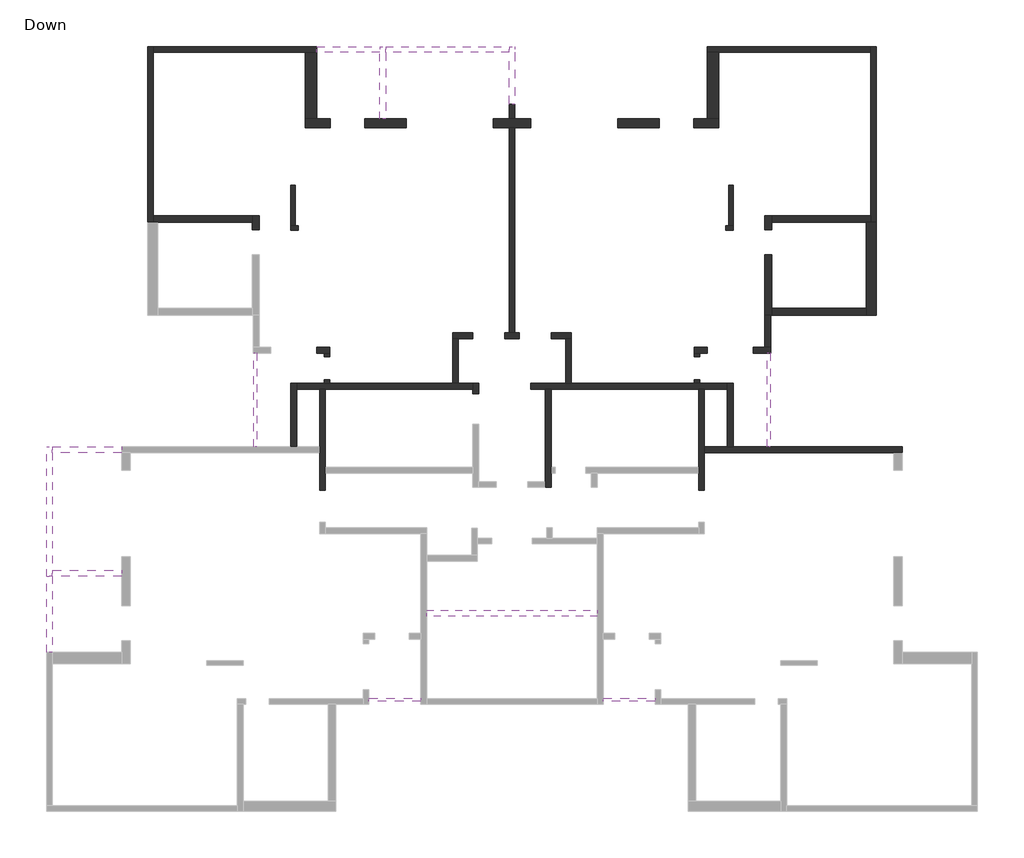
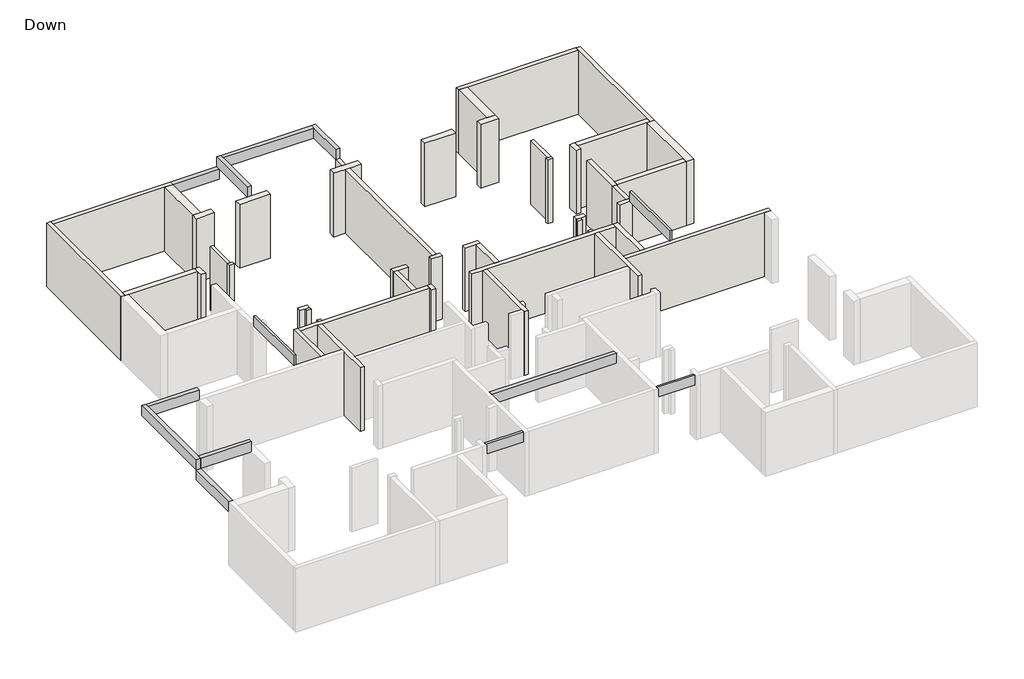
# One storey, part 2 of 2: 46 walls, 13 beams.
"""IFC4 building model written with IfcOpenShell, lengths in millimetres."""

from ifc_helpers import new_model, si_unit, frame, origin, place, context, project, spatial, polyline, outline, extrude, faceted_brep, element, save

model = new_model("IFC4")

# Units and contexts
model_context = context("Model", 3, world=origin())
ifc_project = project(units=[si_unit("LENGTHUNIT", "METRE", prefix="MILLI")], contexts=[model_context])

# Site, building, storey
site = spatial("IfcSite", under=ifc_project)
building = spatial("IfcBuilding", under=site)
storey = spatial("IfcBuildingStorey", under=building, Name="Down", Elevation=0.0)

# Beams
placement = place(None, origin())
element("IfcBeam", 1, ObjectType="Concrete Rectengular Beam : 10/50", at=placement, inside=storey, context=model_context, shape_type="Brep", body=[
    faceted_brep([(-4793.2776511, -8420.9452063, 3180.0), (-4793.2776511, -8520.9452063, 3180.0), (-2993.9832015, -8520.9452063, 3180.0), (-2993.9832015, -8420.9452063, 3180.0), (-4793.2776511, -8520.9452063, 2680.0), (-2993.9832015, -8520.9452063, 2680.0), (-4793.2776511, -8420.9452063, 2680.0), (-2993.9832015, -8420.9452063, 2680.0), (-4793.2776511, -8420.9452063, 2980.0), (-2993.9832015, -8420.9452063, 2980.0)], [[[0, 1, 2, 3]], [[1, 4, 5, 2]], [[4, 6, 7, 5]], [[6, 8, 0, 3, 9, 7]], [[1, 0, 8, 6, 4]], [[3, 2, 5, 7, 9]]]),
])
element("IfcBeam", 2, ObjectType="Concrete Rectengular Beam : 10/50", at=placement, inside=storey, context=model_context, shape_type="Brep", body=[
    faceted_brep([(3308.0864128, -8420.9495778, 3180.0), (3308.0864128, -8520.9495778, 3180.0), (5107.3808625, -8520.9495778, 3180.0), (5107.3808625, -8420.9495778, 3180.0), (3308.0864128, -8520.9495778, 2680.0), (5107.3808625, -8520.9495778, 2680.0), (3308.0864128, -8420.9495778, 2680.0), (5107.3808625, -8420.9495778, 2680.0), (3308.0864128, -8420.9495778, 2980.0), (5107.3808625, -8420.9495778, 2980.0)], [[[0, 1, 2, 3]], [[1, 4, 5, 2]], [[4, 6, 7, 5]], [[6, 8, 0, 3, 9, 7]], [[1, 0, 8, 6, 4]], [[3, 2, 5, 7, 9]]]),
])
element("IfcBeam", 3, ObjectType="Concrete Rectengular Beam : 10/50", at=placement, inside=storey, context=model_context, shape_type="SweptSolid", body=[
    extrude(outline(polyline([(-8674.1337189, 279.007757), (-8774.1337189, 279.007757), (-8774.1337189, 3529.1488671), (-8674.1337189, 3529.1488671), (-8674.1337189, 279.007757)])), frame((0.0, 0.0, 3180.0), z_axis=(0.0, 0.0, 1.0), x_axis=(1.0, 0.0, 0.0)), (0.0, 0.0, 1.0), 500.0),
])
element("IfcBeam", 4, ObjectType="Concrete Rectengular Beam : 10/50", at=placement, inside=storey, context=model_context, shape_type="SweptSolid", body=[
    extrude(outline(polyline([(9086.6847195, 279.007757), (8986.6847195, 279.007757), (8986.6847195, 3529.1488671), (9086.6847195, 3529.1488671), (9086.6847195, 279.007757)])), frame((0.0, 0.0, 3180.0), z_axis=(0.0, 0.0, 1.0), x_axis=(1.0, 0.0, 0.0)), (0.0, 0.0, 1.0), 500.0),
])
element("IfcBeam", 5, ObjectType="Concrete Rectengular Beam : 20/50", at=placement, inside=storey, context=model_context, shape_type="Brep", body=[
    faceted_brep([(57.0516057, 12129.1018304, 3680.0), (57.0516057, 12129.1018304, 3180.0), (257.0516057, 12129.1018304, 3180.0), (257.0516057, 12129.1018304, 3680.0), (257.0516057, 13929.1018304, 3680.0), (257.0516057, 14129.1018304, 3680.0), (57.0516057, 14129.1018304, 3680.0), (57.0516057, 13929.1018304, 3680.0), (257.0516057, 13929.1018304, 3180.0), (257.0516057, 14129.1018304, 3180.0), (57.0516057, 13929.1018304, 3180.0), (57.0516057, 14129.1018304, 3180.0)], [[[0, 1, 2, 3]], [[0, 3, 4, 5, 6, 7]], [[3, 2, 8, 9, 5, 4]], [[2, 1, 10, 11, 9, 8]], [[1, 0, 7, 6, 11, 10]], [[6, 5, 9, 11]]]),
])
element("IfcBeam", 6, ObjectType="Concrete Rectengular Beam : 20/50", at=placement, inside=storey, context=model_context, shape_type="SweptSolid", body=[
    extrude(outline(polyline([(-4213.3152805, 13929.1018304), (-4213.3152805, 14129.1018304), (57.0516057, 14129.1018304), (57.0516057, 13929.1018304), (-4213.3152805, 13929.1018304)])), frame((0.0, 0.0, 3180.0), z_axis=(0.0, 0.0, 1.0), x_axis=(1.0, 0.0, 0.0)), (0.0, 0.0, 1.0), 500.0),
])
element("IfcBeam", 7, ObjectType="Concrete Rectengular Beam : 20/50", at=placement, inside=storey, context=model_context, shape_type="Brep", body=[
    faceted_brep([(-4213.3152805, 11629.007757, 3680.0), (-4413.3152805, 11629.007757, 3680.0), (-4413.3152805, 11629.007757, 3180.0), (-4213.3152805, 11629.007757, 3180.0), (-4213.3152805, 14129.1018304, 3680.0), (-4213.3152805, 14129.1018304, 3180.0), (-4413.3152805, 14129.1018304, 3180.0), (-4413.3152805, 14129.1018304, 3680.0), (-4213.3152805, 13929.1018304, 3680.0), (-4213.3152805, 13929.1018304, 3180.0)], [[[0, 1, 2, 3]], [[4, 5, 6, 7]], [[1, 0, 8, 4, 7]], [[2, 1, 7, 6]], [[3, 2, 6, 5, 9]], [[0, 3, 9, 5, 4, 8]]]),
])
element("IfcBeam", 8, ObjectType="Concrete Rectengular Beam : 20/50", at=placement, inside=storey, context=model_context, shape_type="Brep", body=[
    faceted_brep([(-15942.7132109, -4192.3939363, 3180.0), (-15742.7132109, -4192.3939363, 3180.0), (-15742.7132109, -4192.3939363, 2680.0), (-15942.7132109, -4192.3939363, 2680.0), (-15942.7132109, -4192.3939363, 2980.0), (-15942.7132109, -6821.2744631, 3180.0), (-15742.7132109, -6821.2744631, 3180.0), (-15742.7132109, -6821.2744631, 2680.0), (-15942.7132109, -6821.2744631, 2680.0)], [[[0, 1, 2, 3, 4]], [[1, 0, 5, 6]], [[2, 1, 6, 7]], [[3, 2, 7, 8]], [[0, 4, 3, 8, 5]], [[6, 5, 8, 7]]]),
])
element("IfcBeam", 9, ObjectType="Concrete Rectengular Beam : 20/50", at=placement, inside=storey, context=model_context, shape_type="SweptSolid", body=[
    extrude(outline(polyline([(-13342.9013576, -3992.3939363), (-13342.9013576, -4192.3939363), (-15742.7132109, -4192.3939363), (-15742.7132109, -3992.3939363), (-13342.9013576, -3992.3939363)])), frame((0.0, 0.0, 3180.0), z_axis=(0.0, 0.0, 1.0), x_axis=(1.0, 0.0, 0.0)), (0.0, 0.0, 1.0), 500.0),
])
element("IfcBeam", 10, ObjectType="Concrete Rectengular Beam : 20/50", at=placement, inside=storey, context=model_context, shape_type="Brep", body=[
    faceted_brep([(-15942.7132109, -4192.3939363, 3680.0), (-15942.7132109, -4192.3939363, 3180.0), (-15742.7132109, -4192.3939363, 3180.0), (-15742.7132109, -4192.3939363, 3680.0), (-15742.7132109, -3992.3939363, 3680.0), (-15742.7132109, 79.007757, 3680.0), (-15742.7132109, 279.007757, 3680.0), (-15942.7132109, 279.007757, 3680.0), (-15742.7132109, -3992.3939363, 3180.0), (-15742.7132109, 79.007757, 3180.0), (-15742.7132109, 279.007757, 3180.0), (-15942.7132109, 279.007757, 3180.0)], [[[0, 1, 2, 3]], [[0, 3, 4, 5, 6, 7]], [[3, 2, 8, 9, 10, 6, 5, 4]], [[2, 1, 11, 10, 9, 8]], [[1, 0, 7, 11]], [[7, 6, 10, 11]]]),
])
element("IfcBeam", 11, ObjectType="Concrete Rectengular Beam : 20/50", at=placement, inside=storey, context=model_context, shape_type="SweptSolid", body=[
    extrude(outline(polyline([(-13343.4657979, 279.007757), (-13343.4657979, 79.007757), (-15742.7132109, 79.007757), (-15742.7132109, 279.007757), (-13343.4657979, 279.007757)])), frame((0.0, 0.0, 3180.0), z_axis=(0.0, 0.0, 1.0), x_axis=(1.0, 0.0, 0.0)), (0.0, 0.0, 1.0), 500.0),
])
element("IfcBeam", 12, ObjectType="Concrete Rectengular Beam : 20/50", at=placement, inside=storey, context=model_context, shape_type="Brep", body=[
    faceted_brep([(-4413.3152805, 13929.1018304, 3180.0), (-4413.3152805, 13929.1018304, 2680.0), (-4413.3152805, 14129.1018304, 2680.0), (-4413.3152805, 14129.1018304, 2980.0), (-4413.3152805, 14129.1018304, 3180.0), (-6593.4657979, 14129.1018304, 3180.0), (-6593.4657979, 13929.3370139, 3180.0), (-6593.4657979, 13929.1018304, 3180.0), (-6593.4657979, 14129.1018304, 2680.0), (-6593.4657979, 13929.1018304, 2680.0)], [[[0, 1, 2, 3, 4]], [[0, 4, 5, 6, 7]], [[4, 3, 2, 8, 5]], [[2, 1, 9, 8]], [[1, 0, 7, 9]], [[5, 8, 9, 7, 6]]]),
])
element("IfcBeam", 13, ObjectType="Concrete Rectengular Beam : 20/50", at=placement, inside=storey, context=model_context, shape_type="Brep", body=[
    faceted_brep([(-2793.9832015, -5372.4503803, 3180.0), (-2793.9832015, -5572.4503803, 3180.0), (3108.0864128, -5572.4503803, 3180.0), (3108.0864128, -5372.4503803, 3180.0), (-2793.9832015, -5572.4503803, 2680.0), (3108.0864128, -5572.4503803, 2680.0), (-2793.9832015, -5372.4503803, 2680.0), (3108.0864128, -5372.4503803, 2680.0), (-2793.9832015, -5372.4503803, 2980.0), (3108.0864128, -5372.4503803, 2980.0)], [[[0, 1, 2, 3]], [[1, 4, 5, 2]], [[4, 6, 7, 5]], [[6, 8, 0, 3, 9, 7]], [[1, 0, 8, 6, 4]], [[3, 2, 5, 7, 9]]]),
])

# Walls
element("IfcWall", 14, ObjectType="15", at=placement, inside=storey, context=model_context, shape_type="Brep", body=[
    faceted_brep([(-7241.1610001, 7927.5496197, 0.0), (-7340.9258167, 7927.5496197, 0.0), (-7490.9258167, 7927.5496197, 0.0), (-7490.9258167, 7927.5496197, 3180.0), (-7340.9258167, 7927.5496197, 3180.0), (-7241.1610001, 7927.5496197, 3180.0), (-7241.1610001, 7927.5496197, 2980.0), (-7241.1610001, 7777.5496197, 0.0), (-7241.1610001, 7777.5496197, 2980.0), (-7241.1610001, 7777.5496197, 3180.0), (-7490.9258167, 7777.5496197, 3180.0), (-7490.9258167, 7777.5496197, 2980.0), (-7490.9258167, 7777.5496197, 0.0)], [[[0, 1, 2, 3, 4, 5, 6]], [[7, 8, 9, 10, 11, 12]], [[2, 1, 0, 7, 12]], [[5, 4, 3, 10, 9]], [[0, 6, 5, 9, 8, 7]], [[3, 2, 12, 11, 10]]]),
])
element("IfcWall", 15, ObjectType="15", at=placement, inside=storey, context=model_context, shape_type="Brep", body=[
    faceted_brep([(-7340.9258167, 7927.5496197, 0.0), (-7340.9258167, 9328.7725736, 0.0), (-7340.9258167, 9328.7725736, 2980.0), (-7340.9258167, 9328.7725736, 3180.0), (-7340.9258167, 7927.5496197, 3180.0), (-7340.9258167, 7927.5496197, 2980.0), (-7490.9258167, 7927.5496197, 0.0), (-7490.9258167, 7927.5496197, 3180.0), (-7490.9258167, 9328.7725736, 3180.0), (-7490.9258167, 9328.7725736, 2980.0), (-7490.9258167, 9328.7725736, 0.0)], [[[0, 1, 2, 3, 4, 5]], [[6, 7, 8, 9, 10]], [[1, 0, 6, 10]], [[3, 2, 1, 10, 9, 8]], [[4, 3, 8, 7]], [[0, 5, 4, 7, 6]]]),
])
element("IfcWall", 16, ObjectType="15", at=placement, inside=storey, context=model_context, shape_type="Brep", body=[
    faceted_brep([(7555.2642115, 7777.5496197, 0.0), (7805.0290281, 7777.5496197, 0.0), (7805.0290281, 7777.5496197, 2980.0), (7805.0290281, 7777.5496197, 3180.0), (7555.2642115, 7777.5496197, 3180.0), (7555.2642115, 7777.5496197, 2980.0), (7555.2642115, 7927.5496197, 0.0), (7555.2642115, 7927.5496197, 2980.0), (7555.2642115, 7927.5496197, 3180.0), (7655.0290281, 7927.5496197, 3180.0), (7805.0290281, 7927.5496197, 3180.0), (7805.0290281, 7927.5496197, 0.0), (7655.0290281, 7927.5496197, 0.0)], [[[0, 1, 2, 3, 4, 5]], [[6, 7, 8, 9, 10, 11, 12]], [[1, 0, 6, 12, 11]], [[4, 3, 10, 9, 8]], [[0, 5, 4, 8, 7, 6]], [[3, 2, 1, 11, 10]]]),
])
element("IfcWall", 17, ObjectType="15", at=placement, inside=storey, context=model_context, shape_type="Brep", body=[
    faceted_brep([(7805.0290281, 7927.5496197, 0.0), (7805.0290281, 9328.7725736, 0.0), (7805.0290281, 9328.7725736, 2980.0), (7805.0290281, 9328.7725736, 3180.0), (7805.0290281, 7927.5496197, 3180.0), (7655.0290281, 7927.5496197, 0.0), (7655.0290281, 7927.5496197, 2980.0), (7655.0290281, 7927.5496197, 3180.0), (7655.0290281, 9328.7725736, 3180.0), (7655.0290281, 9328.7725736, 2980.0), (7655.0290281, 9328.7725736, 0.0)], [[[0, 1, 2, 3, 4]], [[5, 6, 7, 8, 9, 10]], [[1, 0, 5, 10]], [[3, 2, 1, 10, 9, 8]], [[4, 3, 8, 7]], [[0, 4, 7, 6, 5]]]),
])
element("IfcWall", 18, ObjectType="20", at=placement, inside=storey, context=model_context, shape_type="Brep", body=[
    faceted_brep([(-12443.8891281, 14129.3370139, 0.0), (-12443.8891281, 8055.2636366, 0.0), (-12443.8891281, 8055.2636366, 3180.0), (-12443.8891281, 14129.3370139, 3180.0), (-12243.8891281, 14129.3370139, 0.0), (-12243.8891281, 14129.3370139, 3180.0), (-12243.8891281, 13929.3370139, 3180.0), (-12243.8891281, 8285.2636366, 3180.0), (-12243.8891281, 8055.2636366, 3180.0), (-12243.8891281, 8055.2636366, 0.0), (-12243.8891281, 8285.2636366, 0.0), (-12243.8891281, 13929.3370139, 0.0)], [[[0, 1, 2, 3]], [[4, 5, 6, 7, 8, 9, 10, 11]], [[1, 0, 4, 11, 10, 9]], [[3, 2, 8, 7, 6, 5]], [[2, 1, 9, 8]], [[0, 3, 5, 4]]]),
])
element("IfcWall", 19, ObjectType="20", at=placement, inside=storey, context=model_context, shape_type="Brep", body=[
    faceted_brep([(-6593.4657979, 3529.1488671, 0.0), (-6344.7357885, 3529.1488671, 0.0), (-6144.7357885, 3529.1488671, 0.0), (-6144.7357885, 3529.1488671, 3180.0), (-6344.7357885, 3529.1488671, 3180.0), (-6593.4657979, 3529.1488671, 3180.0), (-6593.4657979, 3529.1488671, 2980.0), (-6593.4657979, 3729.1488671, 0.0), (-6593.4657979, 3729.1488671, 2980.0), (-6593.4657979, 3729.1488671, 3180.0), (-6144.7357885, 3729.1488671, 3180.0), (-6144.7357885, 3729.1488671, 2980.0), (-6144.7357885, 3729.1488671, 0.0)], [[[0, 1, 2, 3, 4, 5, 6]], [[7, 8, 9, 10, 11, 12]], [[2, 1, 0, 7, 12]], [[5, 4, 3, 10, 9]], [[0, 6, 5, 9, 8, 7]], [[3, 2, 12, 11, 10]]]),
])
element("IfcWall", 20, ObjectType="20", at=placement, inside=storey, context=model_context, shape_type="Brep", body=[
    faceted_brep([(-6344.7357885, 3529.1488671, 0.0), (-6344.7357885, 3397.9165059, 0.0), (-6344.7357885, 3397.9165059, 2980.0), (-6344.7357885, 3397.9165059, 3180.0), (-6344.7357885, 3529.1488671, 3180.0), (-6344.7357885, 3529.1488671, 2980.0), (-6144.7357885, 3529.1488671, 0.0), (-6144.7357885, 3529.1488671, 3180.0), (-6144.7357885, 3397.9165059, 3180.0), (-6144.7357885, 3397.9165059, 2980.0), (-6144.7357885, 3397.9165059, 0.0)], [[[0, 1, 2, 3, 4, 5]], [[6, 7, 8, 9, 10]], [[1, 0, 6, 10]], [[3, 2, 1, 10, 9, 8]], [[4, 3, 8, 7]], [[0, 5, 4, 7, 6]]]),
])
element("IfcWall", 21, ObjectType="20", at=placement, inside=storey, context=model_context, shape_type="Brep", body=[
    faceted_brep([(-6344.7357885, 2597.8224325, 0.0), (-6344.7357885, 2479.2899772, 0.0), (-6344.7357885, 2479.2899772, 2980.0), (-6344.7357885, 2479.2899772, 3180.0), (-6344.7357885, 2597.8224325, 3180.0), (-6344.7357885, 2597.8224325, 2980.0), (-6144.7357885, 2597.8224325, 0.0), (-6144.7357885, 2597.8224325, 2980.0), (-6144.7357885, 2597.8224325, 3180.0), (-6144.7357885, 2479.2899772, 3180.0), (-6144.7357885, 2479.2899772, 2980.0), (-6144.7357885, 2479.2899772, 0.0)], [[[0, 1, 2, 3, 4, 5]], [[6, 7, 8, 9, 10, 11]], [[1, 0, 6, 11]], [[4, 3, 9, 8]], [[0, 5, 4, 8, 7, 6]], [[3, 2, 1, 11, 10, 9]]]),
])
element("IfcWall", 22, ObjectType="20", at=placement, inside=storey, context=model_context, shape_type="Brep", body=[
    faceted_brep([(-7293.0424677, 2279.2899772, 0.0), (-6495.0180086, 2279.2899772, 0.0), (-6295.0180086, 2279.2899772, 0.0), (-1194.9239352, 2279.2899772, 0.0), (-1194.9239352, 2279.2899772, 3180.0), (-6295.0180086, 2279.2899772, 3180.0), (-6495.0180086, 2279.2899772, 3180.0), (-7293.0424677, 2279.2899772, 3180.0), (-7293.0424677, 2479.2899772, 0.0), (-7293.0424677, 2479.2899772, 3180.0), (-6344.7357885, 2479.2899772, 3180.0), (-6144.7357885, 2479.2899772, 3180.0), (-1894.500605, 2479.2899772, 3180.0), (-1694.500605, 2479.2899772, 3180.0), (-1194.9239352, 2479.2899772, 3180.0), (-1194.9239352, 2479.2899772, 0.0), (-1694.500605, 2479.2899772, 0.0), (-1894.500605, 2479.2899772, 0.0), (-6144.7357885, 2479.2899772, 0.0), (-6344.7357885, 2479.2899772, 0.0)], [[[0, 1, 2, 3, 4, 5, 6, 7]], [[8, 9, 10, 11, 12, 13, 14, 15, 16, 17, 18, 19]], [[3, 2, 1, 0, 8, 19, 18, 17, 16, 15]], [[7, 6, 5, 4, 14, 13, 12, 11, 10, 9]], [[4, 3, 15, 14]], [[0, 7, 9, 8]]]),
])
element("IfcWall", 23, ObjectType="20", at=placement, inside=storey, context=model_context, shape_type="Brep", body=[
    faceted_brep([(-1194.9239352, 2479.2899772, 0.0), (-1194.9239352, 2279.2899772, 0.0), (-1194.9239352, 2127.9259132, 0.0), (-1194.9239352, 2127.9259132, 2980.0), (-1194.9239352, 2127.9259132, 3180.0), (-1194.9239352, 2279.2899772, 3180.0), (-1194.9239352, 2479.2899772, 3180.0), (-994.9239352, 2479.2899772, 0.0), (-994.9239352, 2479.2899772, 2980.0), (-994.9239352, 2479.2899772, 3180.0), (-994.9239352, 2127.9259132, 3180.0), (-994.9239352, 2127.9259132, 2980.0), (-994.9239352, 2127.9259132, 0.0), (-1133.7398977, 2479.2899772, 3180.0)], [[[0, 1, 2, 3, 4, 5, 6]], [[7, 8, 9, 10, 11, 12]], [[2, 1, 0, 7, 12]], [[4, 3, 2, 12, 11, 10]], [[6, 5, 4, 10, 9, 13]], [[0, 6, 13, 9, 8, 7]]]),
])
element("IfcWall", 24, ObjectType="20", at=placement, inside=storey, context=model_context, shape_type="Brep", body=[
    faceted_brep([(-6295.0180086, -1222.7326004, 0.0), (-6295.0180086, -621.6037199, 0.0), (-6295.0180086, -421.6037199, 0.0), (-6295.0180086, 2279.2899772, 0.0), (-6295.0180086, 2279.2899772, 3180.0), (-6295.0180086, -421.6037199, 3180.0), (-6295.0180086, -621.6037199, 3180.0), (-6295.0180086, -1222.7326004, 3180.0), (-6295.0180086, -1222.7326004, 2980.0), (-6495.0180086, -1222.7326004, 0.0), (-6495.0180086, -1222.7326004, 2980.0), (-6495.0180086, -1222.7326004, 3180.0), (-6495.0180086, 79.007757, 3180.0), (-6495.0180086, 279.007757, 3180.0), (-6495.0180086, 2279.2899772, 3180.0), (-6495.0180086, 2279.2899772, 0.0), (-6495.0180086, 279.007757, 0.0), (-6495.0180086, 79.007757, 0.0)], [[[0, 1, 2, 3, 4, 5, 6, 7, 8]], [[9, 10, 11, 12, 13, 14, 15, 16, 17]], [[3, 2, 1, 0, 9, 17, 16, 15]], [[7, 6, 5, 4, 14, 13, 12, 11]], [[0, 8, 7, 11, 10, 9]], [[4, 3, 15, 14]]]),
])
element("IfcWall", 25, ObjectType="20", at=placement, inside=storey, context=model_context, shape_type="Brep", body=[
    faceted_brep([(-7493.0424677, 2479.2899772, 0.0), (-7493.0424677, 279.007757, 0.0), (-7493.0424677, 279.007757, 2980.0), (-7493.0424677, 279.007757, 3180.0), (-7493.0424677, 2479.2899772, 3180.0), (-7493.0424677, 2479.2899772, 2980.0), (-7293.0424677, 2479.2899772, 0.0), (-7293.0424677, 2479.2899772, 3180.0), (-7293.0424677, 2279.2899772, 3180.0), (-7293.0424677, 279.007757, 3180.0), (-7293.0424677, 279.007757, 0.0), (-7293.0424677, 2279.2899772, 0.0)], [[[0, 1, 2, 3, 4, 5]], [[6, 7, 8, 9, 10, 11]], [[1, 0, 6, 11, 10]], [[4, 3, 9, 8, 7]], [[3, 2, 1, 10, 9]], [[0, 5, 4, 7, 6]]]),
])
element("IfcWall", 26, ObjectType="20", at=placement, inside=storey, context=model_context, shape_type="Brep", body=[
    faceted_brep([(-12243.8891281, 13929.3370139, 0.0), (-6993.4657979, 13929.3370139, 0.0), (-6593.4657979, 13929.3370139, 0.0), (-6593.4657979, 13929.3370139, 3180.0), (-6993.4657979, 13929.3370139, 3180.0), (-12243.8891281, 13929.3370139, 3180.0), (-12243.8891281, 13929.3370139, 2980.0), (-12243.8891281, 14129.3370139, 0.0), (-12243.8891281, 14129.3370139, 3180.0), (-6593.4657979, 14129.3370139, 3180.0), (-6593.4657979, 14129.3370139, 0.0), (-6593.4657979, 14129.1018304, 3180.0)], [[[0, 1, 2, 3, 4, 5, 6]], [[7, 8, 9, 10]], [[2, 1, 0, 7, 10]], [[5, 4, 3, 11, 9, 8]], [[0, 6, 5, 8, 7]], [[3, 2, 10, 9, 11]]]),
])
element("IfcWall", 27, ObjectType="20", at=placement, inside=storey, context=model_context, shape_type="Brep", body=[
    faceted_brep([(57.0516057, 12129.1018304, 0.0), (57.0516057, 11629.007757, 0.0), (57.0516057, 11629.007757, 2980.0), (57.0516057, 11629.007757, 3180.0), (57.0516057, 12129.1018304, 3180.0), (57.0516057, 12129.1018304, 2980.0), (257.0516057, 12129.1018304, 0.0), (257.0516057, 12129.1018304, 2980.0), (257.0516057, 12129.1018304, 3180.0), (257.0516057, 11629.007757, 3180.0), (257.0516057, 11629.007757, 2980.0), (257.0516057, 11629.007757, 0.0)], [[[0, 1, 2, 3, 4, 5]], [[6, 7, 8, 9, 10, 11]], [[1, 0, 6, 11]], [[4, 3, 9, 8]], [[0, 5, 4, 8, 7, 6]], [[3, 2, 1, 11, 10, 9]]]),
])
element("IfcWall", 28, ObjectType="20", at=placement, inside=storey, context=model_context, shape_type="Brep", body=[
    faceted_brep([(57.0516057, 11329.007757, 0.0), (57.0516057, 4229.007757, 0.0), (57.0516057, 4229.007757, 2980.0), (57.0516057, 4229.007757, 3180.0), (57.0516057, 11329.007757, 3180.0), (57.0516057, 11329.007757, 2980.0), (257.0516057, 11329.007757, 0.0), (257.0516057, 11329.007757, 2980.0), (257.0516057, 11329.007757, 3180.0), (257.0516057, 4229.007757, 3180.0), (257.0516057, 4229.007757, 2980.0), (257.0516057, 4229.007757, 0.0)], [[[0, 1, 2, 3, 4, 5]], [[6, 7, 8, 9, 10, 11]], [[1, 0, 6, 11]], [[4, 3, 9, 8]], [[0, 5, 4, 8, 7, 6]], [[3, 2, 1, 11, 10, 9]]]),
])
element("IfcWall", 29, ObjectType="20", at=placement, inside=storey, context=model_context, shape_type="Brep", body=[
    faceted_brep([(407.3338258, 4229.007757, 0.0), (257.0516057, 4229.007757, 0.0), (57.0516057, 4229.007757, 0.0), (-93.2306144, 4229.007757, 0.0), (-93.2306144, 4229.007757, 2980.0), (-93.2306144, 4229.007757, 3180.0), (57.0516057, 4229.007757, 3180.0), (257.0516057, 4229.007757, 3180.0), (407.3338258, 4229.007757, 3180.0), (407.3338258, 4229.007757, 2980.0), (407.3338258, 4029.007757, 0.0), (407.3338258, 4029.007757, 2980.0), (407.3338258, 4029.007757, 3180.0), (-93.2306144, 4029.007757, 3180.0), (-93.2306144, 4029.007757, 2980.0), (-93.2306144, 4029.007757, 0.0)], [[[0, 1, 2, 3, 4, 5, 6, 7, 8, 9]], [[10, 11, 12, 13, 14, 15]], [[3, 2, 1, 0, 10, 15]], [[5, 4, 3, 15, 14, 13]], [[8, 7, 6, 5, 13, 12]], [[0, 9, 8, 12, 11, 10]]]),
])
element("IfcWall", 30, ObjectType="20", at=placement, inside=storey, context=model_context, shape_type="Brep", body=[
    faceted_brep([(-1193.8891281, 4228.6785002, 0.0), (-1894.500605, 4228.6785002, 0.0), (-1894.500605, 4228.6785002, 2980.0), (-1894.500605, 4228.6785002, 3180.0), (-1193.8891281, 4228.6785002, 3180.0), (-1193.8891281, 4228.6785002, 2980.0), (-1193.8891281, 4028.6785002, 0.0), (-1193.8891281, 4028.6785002, 3180.0), (-1694.500605, 4028.6785002, 3180.0), (-1894.500605, 4028.6785002, 3180.0), (-1894.500605, 4028.6785002, 0.0), (-1694.500605, 4028.6785002, 0.0), (-1193.8891281, 4029.007757, 3180.0)], [[[0, 1, 2, 3, 4, 5]], [[6, 7, 8, 9, 10, 11]], [[1, 0, 6, 11, 10]], [[4, 3, 9, 8, 7, 12]], [[0, 5, 4, 12, 7, 6]], [[3, 2, 1, 10, 9]]]),
])
element("IfcWall", 31, ObjectType="20", at=placement, inside=storey, context=model_context, shape_type="Brep", body=[
    faceted_brep([(-1894.500605, 4028.6785002, 0.0), (-1894.500605, 2479.2899772, 0.0), (-1894.500605, 2479.2899772, 2980.0), (-1894.500605, 2479.2899772, 3180.0), (-1894.500605, 4028.6785002, 3180.0), (-1694.500605, 4028.6785002, 0.0), (-1694.500605, 4028.6785002, 3180.0), (-1694.500605, 2479.2899772, 3180.0), (-1694.500605, 2479.2899772, 0.0)], [[[0, 1, 2, 3, 4]], [[5, 6, 7, 8]], [[1, 0, 5, 8]], [[4, 3, 7, 6]], [[0, 4, 6, 5]], [[3, 2, 1, 8, 7]]]),
])
element("IfcWall", 32, ObjectType="20", at=placement, inside=storey, context=model_context, shape_type="Brep", body=[
    faceted_brep([(12557.9923395, 14129.3370139, 0.0), (12557.9923395, 13929.3370139, 0.0), (12557.9923395, 8285.2636366, 0.0), (12557.9923395, 8055.2636366, 0.0), (12557.9923395, 8055.2636366, 3180.0), (12557.9923395, 8285.2636366, 3180.0), (12557.9923395, 13929.3370139, 3180.0), (12557.9923395, 14129.3370139, 3180.0), (12757.9923395, 14129.3370139, 0.0), (12757.9923395, 14129.3370139, 3180.0), (12757.9923395, 8055.2636366, 3180.0), (12757.9923395, 8055.2636366, 0.0)], [[[0, 1, 2, 3, 4, 5, 6, 7]], [[8, 9, 10, 11]], [[3, 2, 1, 0, 8, 11]], [[7, 6, 5, 4, 10, 9]], [[4, 3, 11, 10]], [[0, 7, 9, 8]]]),
])
element("IfcWall", 33, ObjectType="20", at=placement, inside=storey, context=model_context, shape_type="Brep", body=[
    faceted_brep([(8907.8041927, 4828.7725736, 0.0), (8907.8041927, 3729.1488671, 0.0), (8907.8041927, 3729.1488671, 2980.0), (8907.8041927, 3729.1488671, 3180.0), (8907.8041927, 4828.7725736, 3180.0), (9107.8041927, 4828.7725736, 0.0), (9107.8041927, 4828.7725736, 3180.0), (9107.8041927, 3729.1488671, 3180.0), (9107.8041927, 3729.1488671, 0.0)], [[[0, 1, 2, 3, 4]], [[5, 6, 7, 8]], [[1, 0, 5, 8]], [[4, 3, 7, 6]], [[0, 4, 6, 5]], [[3, 2, 1, 8, 7]]]),
])
element("IfcWall", 34, ObjectType="20", at=placement, inside=storey, context=model_context, shape_type="Brep", body=[
    faceted_brep([(9107.8041927, 3729.1488671, 0.0), (8907.8041927, 3729.1488671, 0.0), (8507.757156, 3729.1488671, 0.0), (8507.757156, 3729.1488671, 2980.0), (8507.757156, 3729.1488671, 3180.0), (8907.8041927, 3729.1488671, 3180.0), (9107.8041927, 3729.1488671, 3180.0), (9107.8041927, 3529.1488671, 0.0), (9107.8041927, 3529.1488671, 3180.0), (9086.6847195, 3529.1488671, 3180.0), (8507.757156, 3529.1488671, 3180.0), (8507.757156, 3529.1488671, 2980.0), (8507.757156, 3529.1488671, 0.0)], [[[0, 1, 2, 3, 4, 5, 6]], [[7, 8, 9, 10, 11, 12]], [[2, 1, 0, 7, 12]], [[4, 3, 2, 12, 11, 10]], [[6, 5, 4, 10, 9, 8]], [[0, 6, 8, 7]]]),
])
element("IfcWall", 35, ObjectType="20", at=placement, inside=storey, context=model_context, shape_type="Brep", body=[
    faceted_brep([(6907.5690093, 3729.1488671, 0.0), (6458.8389999, 3729.1488671, 0.0), (6458.8389999, 3729.1488671, 2980.0), (6458.8389999, 3729.1488671, 3180.0), (6907.5690093, 3729.1488671, 3180.0), (6907.5690093, 3729.1488671, 2980.0), (6907.5690093, 3529.1488671, 0.0), (6907.5690093, 3529.1488671, 2980.0), (6907.5690093, 3529.1488671, 3180.0), (6658.8389999, 3529.1488671, 3180.0), (6458.8389999, 3529.1488671, 3180.0), (6458.8389999, 3529.1488671, 0.0), (6658.8389999, 3529.1488671, 0.0)], [[[0, 1, 2, 3, 4, 5]], [[6, 7, 8, 9, 10, 11, 12]], [[1, 0, 6, 12, 11]], [[4, 3, 10, 9, 8]], [[0, 5, 4, 8, 7, 6]], [[3, 2, 1, 11, 10]]]),
])
element("IfcWall", 36, ObjectType="20", at=placement, inside=storey, context=model_context, shape_type="Brep", body=[
    faceted_brep([(6458.8389999, 3529.1488671, 0.0), (6458.8389999, 3397.9165059, 0.0), (6458.8389999, 3397.9165059, 2980.0), (6458.8389999, 3397.9165059, 3180.0), (6458.8389999, 3529.1488671, 3180.0), (6658.8389999, 3529.1488671, 0.0), (6658.8389999, 3529.1488671, 2980.0), (6658.8389999, 3529.1488671, 3180.0), (6658.8389999, 3397.9165059, 3180.0), (6658.8389999, 3397.9165059, 2980.0), (6658.8389999, 3397.9165059, 0.0)], [[[0, 1, 2, 3, 4]], [[5, 6, 7, 8, 9, 10]], [[1, 0, 5, 10]], [[3, 2, 1, 10, 9, 8]], [[4, 3, 8, 7]], [[0, 4, 7, 6, 5]]]),
])
element("IfcWall", 37, ObjectType="20", at=placement, inside=storey, context=model_context, shape_type="Brep", body=[
    faceted_brep([(6458.8389999, 2597.8224325, 0.0), (6458.8389999, 2479.2899772, 0.0), (6458.8389999, 2479.2899772, 2980.0), (6458.8389999, 2479.2899772, 3180.0), (6458.8389999, 2597.8224325, 3180.0), (6458.8389999, 2597.8224325, 2980.0), (6658.8389999, 2597.8224325, 0.0), (6658.8389999, 2597.8224325, 2980.0), (6658.8389999, 2597.8224325, 3180.0), (6658.8389999, 2479.2899772, 3180.0), (6658.8389999, 2479.2899772, 2980.0), (6658.8389999, 2479.2899772, 0.0)], [[[0, 1, 2, 3, 4, 5]], [[6, 7, 8, 9, 10, 11]], [[1, 0, 6, 11]], [[4, 3, 9, 8]], [[0, 5, 4, 8, 7, 6]], [[3, 2, 1, 11, 10, 9]]]),
])
element("IfcWall", 38, ObjectType="20", at=placement, inside=storey, context=model_context, shape_type="Brep", body=[
    faceted_brep([(7607.1456791, 2479.2899772, 0.0), (6658.8389999, 2479.2899772, 0.0), (6458.8389999, 2479.2899772, 0.0), (2208.6038164, 2479.2899772, 0.0), (2008.6038164, 2479.2899772, 0.0), (806.3460554, 2479.2899772, 0.0), (806.3460554, 2479.2899772, 2980.0), (806.3460554, 2479.2899772, 3180.0), (1446.2601023, 2479.2899772, 3180.0), (2008.6038164, 2479.2899772, 3180.0), (2208.6038164, 2479.2899772, 3180.0), (6458.8389999, 2479.2899772, 3180.0), (6658.8389999, 2479.2899772, 3180.0), (7607.1456791, 2479.2899772, 3180.0), (7607.1456791, 2279.2899772, 0.0), (7607.1456791, 2279.2899772, 3180.0), (6809.12122, 2279.2899772, 3180.0), (6609.12122, 2279.2899772, 3180.0), (1509.0271466, 2279.2899772, 3180.0), (1309.0271466, 2279.2899772, 3180.0), (806.3460554, 2279.2899772, 3180.0), (806.3460554, 2279.2899772, 2980.0), (806.3460554, 2279.2899772, 0.0), (1309.0271466, 2279.2899772, 0.0), (1509.0271466, 2279.2899772, 0.0), (6609.12122, 2279.2899772, 0.0), (6809.12122, 2279.2899772, 0.0)], [[[0, 1, 2, 3, 4, 5, 6, 7, 8, 9, 10, 11, 12, 13]], [[14, 15, 16, 17, 18, 19, 20, 21, 22, 23, 24, 25, 26]], [[5, 4, 3, 2, 1, 0, 14, 26, 25, 24, 23, 22]], [[7, 6, 5, 22, 21, 20]], [[13, 12, 11, 10, 9, 8, 7, 20, 19, 18, 17, 16, 15]], [[0, 13, 15, 14]]]),
])
element("IfcWall", 39, ObjectType="20", at=placement, inside=storey, context=model_context, shape_type="Brep", body=[
    faceted_brep([(1309.0271466, 2279.2899772, 0.0), (1309.0271466, -921.133353, 0.0), (1309.0271466, -1121.133353, 0.0), (1309.0271466, -1121.133353, 3180.0), (1309.0271466, -921.133353, 3180.0), (1309.0271466, 2279.2899772, 3180.0), (1309.0271466, 2279.2899772, 2980.0), (1509.0271466, 2279.2899772, 0.0), (1509.0271466, 2279.2899772, 3180.0), (1509.0271466, -422.6385271, 3180.0), (1509.0271466, -622.6385271, 3180.0), (1509.0271466, -1121.133353, 3180.0), (1509.0271466, -1121.133353, 2980.0), (1509.0271466, -1121.133353, 0.0), (1509.0271466, -622.6385271, 0.0), (1509.0271466, -422.6385271, 0.0)], [[[0, 1, 2, 3, 4, 5, 6]], [[7, 8, 9, 10, 11, 12, 13, 14, 15]], [[2, 1, 0, 7, 15, 14, 13]], [[5, 4, 3, 11, 10, 9, 8]], [[0, 6, 5, 8, 7]], [[3, 2, 13, 12, 11]]]),
])
element("IfcWall", 40, ObjectType="20", at=placement, inside=storey, context=model_context, shape_type="Brep", body=[
    faceted_brep([(6809.12122, -1222.7326004, 0.0), (6809.12122, 79.007757, 0.0), (6809.12122, 279.007757, 0.0), (6809.12122, 2279.2899772, 0.0), (6809.12122, 2279.2899772, 3180.0), (6809.12122, 279.007757, 3180.0), (6809.12122, 79.007757, 3180.0), (6809.12122, -1222.7326004, 3180.0), (6809.12122, -1222.7326004, 2980.0), (6609.12122, -1222.7326004, 0.0), (6609.12122, -1222.7326004, 2980.0), (6609.12122, -1222.7326004, 3180.0), (6609.12122, -621.6037199, 3180.0), (6609.12122, -421.6037199, 3180.0), (6609.12122, 2279.2899772, 3180.0), (6609.12122, 2279.2899772, 0.0), (6609.12122, -421.6037199, 0.0), (6609.12122, -621.6037199, 0.0)], [[[0, 1, 2, 3, 4, 5, 6, 7, 8]], [[9, 10, 11, 12, 13, 14, 15, 16, 17]], [[3, 2, 1, 0, 9, 17, 16, 15]], [[7, 6, 5, 4, 14, 13, 12, 11]], [[0, 8, 7, 11, 10, 9]], [[4, 3, 15, 14]]]),
])
element("IfcWall", 41, ObjectType="20", at=placement, inside=storey, context=model_context, shape_type="Brep", body=[
    faceted_brep([(7607.1456791, 2479.2899772, 0.0), (7607.1456791, 2279.2899772, 0.0), (7607.1456791, 279.007757, 0.0), (7607.1456791, 279.007757, 3180.0), (7607.1456791, 2279.2899772, 3180.0), (7607.1456791, 2479.2899772, 3180.0), (7807.1456791, 2479.2899772, 0.0), (7807.1456791, 2479.2899772, 2980.0), (7807.1456791, 2479.2899772, 3180.0), (7807.1456791, 279.007757, 3180.0), (7807.1456791, 279.007757, 2980.0), (7807.1456791, 279.007757, 0.0)], [[[0, 1, 2, 3, 4, 5]], [[6, 7, 8, 9, 10, 11]], [[2, 1, 0, 6, 11]], [[5, 4, 3, 9, 8]], [[3, 2, 11, 10, 9]], [[0, 5, 8, 7, 6]]]),
])
element("IfcWall", 42, ObjectType="20", at=placement, inside=storey, context=model_context, shape_type="Brep", body=[
    faceted_brep([(6809.12122, 79.007757, 0.0), (13357.004569, 79.007757, 0.0), (13657.004569, 79.007757, 0.0), (13657.5690093, 79.007757, 0.0), (13657.5690093, 79.007757, 2980.0), (13657.5690093, 79.007757, 3180.0), (13657.004569, 79.007757, 3180.0), (13357.004569, 79.007757, 3180.0), (6809.12122, 79.007757, 3180.0), (6809.12122, 79.007757, 2980.0), (6809.12122, 279.007757, 0.0), (6809.12122, 279.007757, 3180.0), (7607.1456791, 279.007757, 3180.0), (7807.1456791, 279.007757, 3180.0), (9086.6847195, 279.007757, 3180.0), (13657.5690093, 279.007757, 3180.0), (13657.5690093, 279.007757, 2980.0), (13657.5690093, 279.007757, 0.0), (7807.1456791, 279.007757, 0.0), (7607.1456791, 279.007757, 0.0)], [[[0, 1, 2, 3, 4, 5, 6, 7, 8, 9]], [[10, 11, 12, 13, 14, 15, 16, 17, 18, 19]], [[3, 2, 1, 0, 10, 19, 18, 17]], [[5, 4, 3, 17, 16, 15]], [[8, 7, 6, 5, 15, 14, 13, 12, 11]], [[0, 9, 8, 11, 10]]]),
])
element("IfcWall", 43, ObjectType="20", at=placement, inside=storey, context=model_context, shape_type="Brep", body=[
    faceted_brep([(12557.9923395, 14129.3370139, 0.0), (6907.5690093, 14129.3370139, 0.0), (6907.5690093, 14129.3370139, 3180.0), (12557.9923395, 14129.3370139, 3180.0), (12557.9923395, 13929.3370139, 0.0), (12557.9923395, 13929.3370139, 2980.0), (12557.9923395, 13929.3370139, 3180.0), (7307.5690093, 13929.3370139, 3180.0), (6907.5690093, 13929.3370139, 3180.0), (6907.5690093, 13929.3370139, 0.0), (7307.5690093, 13929.3370139, 0.0), (6907.5690093, 14129.1018304, 3180.0)], [[[0, 1, 2, 3]], [[4, 5, 6, 7, 8, 9, 10]], [[1, 0, 4, 10, 9]], [[3, 2, 11, 8, 7, 6]], [[0, 3, 6, 5, 4]], [[2, 1, 9, 8, 11]]]),
])
element("IfcWall", 44, ObjectType="20", at=placement, inside=storey, context=model_context, shape_type="Brep", body=[
    faceted_brep([(1507.9923395, 4028.6785002, 0.0), (2008.6038164, 4028.6785002, 0.0), (2208.6038164, 4028.6785002, 0.0), (2208.6038164, 4028.6785002, 3180.0), (2008.6038164, 4028.6785002, 3180.0), (1507.9923395, 4028.6785002, 3180.0), (1507.9923395, 4228.6785002, 0.0), (1507.9923395, 4228.6785002, 2980.0), (1507.9923395, 4228.6785002, 3180.0), (2208.6038164, 4228.6785002, 3180.0), (2208.6038164, 4228.6785002, 2980.0), (2208.6038164, 4228.6785002, 0.0), (1507.9923395, 4029.007757, 3180.0)], [[[0, 1, 2, 3, 4, 5]], [[6, 7, 8, 9, 10, 11]], [[2, 1, 0, 6, 11]], [[5, 4, 3, 9, 8, 12]], [[0, 5, 12, 8, 7, 6]], [[3, 2, 11, 10, 9]]]),
])
element("IfcWall", 45, ObjectType="20", at=placement, inside=storey, context=model_context, shape_type="Brep", body=[
    faceted_brep([(2008.6038164, 4028.6785002, 0.0), (2008.6038164, 2479.2899772, 0.0), (2008.6038164, 2479.2899772, 3180.0), (2008.6038164, 4028.6785002, 3180.0), (2208.6038164, 4028.6785002, 0.0), (2208.6038164, 4028.6785002, 3180.0), (2208.6038164, 2479.2899772, 3180.0), (2208.6038164, 2479.2899772, 2980.0), (2208.6038164, 2479.2899772, 0.0)], [[[0, 1, 2, 3]], [[4, 5, 6, 7, 8]], [[1, 0, 4, 8]], [[3, 2, 6, 5]], [[0, 3, 5, 4]], [[2, 1, 8, 7, 6]]]),
])
element("IfcWall", 46, ObjectType="23", at=placement, inside=storey, context=model_context, shape_type="Brep", body=[
    faceted_brep([(-12243.8891281, 8055.2636366, 0.0), (-12093.8891281, 8055.2636366, 0.0), (-8823.7009813, 8055.2636366, 0.0), (-8823.7009813, 8055.2636366, 2980.0), (-8823.7009813, 8055.2636366, 3180.0), (-12093.8891281, 8055.2636366, 3180.0), (-12243.8891281, 8055.2636366, 3180.0), (-12243.8891281, 8285.2636366, 0.0), (-12243.8891281, 8285.2636366, 2980.0), (-12243.8891281, 8285.2636366, 3180.0), (-8823.7009813, 8285.2636366, 3180.0), (-8823.7009813, 8285.2636366, 0.0)], [[[0, 1, 2, 3, 4, 5, 6]], [[7, 8, 9, 10, 11]], [[2, 1, 0, 7, 11]], [[6, 5, 4, 10, 9]], [[0, 6, 9, 8, 7]], [[4, 3, 2, 11, 10]]]),
])
element("IfcWall", 47, ObjectType="23", at=placement, inside=storey, context=model_context, shape_type="Brep", body=[
    faceted_brep([(-8823.7009813, 8285.2636366, 0.0), (-8823.7009813, 8055.2636366, 0.0), (-8823.7009813, 7785.2636366, 0.0), (-8823.7009813, 7785.2636366, 2980.0), (-8823.7009813, 7785.2636366, 3180.0), (-8823.7009813, 8055.2636366, 3180.0), (-8823.7009813, 8285.2636366, 3180.0), (-8593.7009813, 8285.2636366, 0.0), (-8593.7009813, 8285.2636366, 2980.0), (-8593.7009813, 8285.2636366, 3180.0), (-8593.7009813, 7785.2636366, 3180.0), (-8593.7009813, 7785.2636366, 2980.0), (-8593.7009813, 7785.2636366, 0.0)], [[[0, 1, 2, 3, 4, 5, 6]], [[7, 8, 9, 10, 11, 12]], [[2, 1, 0, 7, 12]], [[4, 3, 2, 12, 11, 10]], [[6, 5, 4, 10, 9]], [[0, 6, 9, 8, 7]]]),
])
element("IfcWall", 48, ObjectType="23", at=placement, inside=storey, context=model_context, shape_type="Brep", body=[
    faceted_brep([(12557.9923395, 8285.2636366, 0.0), (9137.8041927, 8285.2636366, 0.0), (9137.8041927, 8285.2636366, 3180.0), (12557.9923395, 8285.2636366, 3180.0), (12557.9923395, 8285.2636366, 2980.0), (12557.9923395, 8055.2636366, 0.0), (12557.9923395, 8055.2636366, 3180.0), (12407.9923395, 8055.2636366, 3180.0), (9137.8041927, 8055.2636366, 3180.0), (9137.8041927, 8055.2636366, 2980.0), (9137.8041927, 8055.2636366, 0.0), (12407.9923395, 8055.2636366, 0.0)], [[[0, 1, 2, 3, 4]], [[5, 6, 7, 8, 9, 10, 11]], [[1, 0, 5, 11, 10]], [[3, 2, 8, 7, 6]], [[0, 4, 3, 6, 5]], [[2, 1, 10, 9, 8]]]),
])
element("IfcWall", 49, ObjectType="23", at=placement, inside=storey, context=model_context, shape_type="Brep", body=[
    faceted_brep([(8907.8041927, 8285.2636366, 0.0), (8907.8041927, 7785.2636366, 0.0), (8907.8041927, 7785.2636366, 2980.0), (8907.8041927, 7785.2636366, 3180.0), (8907.8041927, 8285.2636366, 3180.0), (8907.8041927, 8285.2636366, 2980.0), (9137.8041927, 8285.2636366, 0.0), (9137.8041927, 8285.2636366, 3180.0), (9137.8041927, 8055.2636366, 3180.0), (9137.8041927, 7785.2636366, 3180.0), (9137.8041927, 7785.2636366, 2980.0), (9137.8041927, 7785.2636366, 0.0), (9137.8041927, 8055.2636366, 0.0)], [[[0, 1, 2, 3, 4, 5]], [[6, 7, 8, 9, 10, 11, 12]], [[1, 0, 6, 12, 11]], [[3, 2, 1, 11, 10, 9]], [[4, 3, 9, 8, 7]], [[0, 5, 4, 7, 6]]]),
])
element("IfcWall", 50, ObjectType="23", at=placement, inside=storey, context=model_context, shape_type="Brep", body=[
    faceted_brep([(8907.8041927, 6932.7236554, 0.0), (8907.8041927, 4828.7725736, 0.0), (8907.8041927, 4828.7725736, 3180.0), (8907.8041927, 6932.7236554, 3180.0), (8907.8041927, 6932.7236554, 2980.0), (9137.8041927, 6932.7236554, 0.0), (9137.8041927, 6932.7236554, 2980.0), (9137.8041927, 6932.7236554, 3180.0), (9137.8041927, 5078.7725736, 3180.0), (9137.8041927, 4828.7725736, 3180.0), (9137.8041927, 4828.7725736, 0.0), (9137.8041927, 5078.7725736, 0.0), (9107.8041927, 4828.7725736, 0.0), (9107.8041927, 4828.7725736, 3180.0)], [[[0, 1, 2, 3, 4]], [[5, 6, 7, 8, 9, 10, 11]], [[1, 0, 5, 11, 10, 12]], [[3, 2, 13, 9, 8, 7]], [[0, 4, 3, 7, 6, 5]], [[2, 1, 12, 10, 9, 13]]]),
])
element("IfcWall", 51, ObjectType="25", at=placement, inside=storey, context=model_context, shape_type="Brep", body=[
    faceted_brep([(12407.9923395, 5078.7725736, 0.0), (9137.8041927, 5078.7725736, 0.0), (9137.8041927, 5078.7725736, 2980.0), (9137.8041927, 5078.7725736, 3180.0), (12407.9923395, 5078.7725736, 3180.0), (12407.9923395, 5078.7725736, 2980.0), (12407.9923395, 4828.7725736, 0.0), (12407.9923395, 4828.7725736, 3180.0), (9137.8041927, 4828.7725736, 3180.0), (9137.8041927, 4828.7725736, 0.0)], [[[0, 1, 2, 3, 4, 5]], [[6, 7, 8, 9]], [[1, 0, 6, 9]], [[4, 3, 8, 7]], [[3, 2, 1, 9, 8]], [[0, 5, 4, 7, 6]]]),
])
element("IfcWall", 52, ObjectType="30", at=placement, inside=storey, context=model_context, shape_type="Brep", body=[
    faceted_brep([(-6993.4657979, 11328.25517, 0.0), (-6133.4657979, 11328.25517, 0.0), (-6133.4657979, 11328.25517, 2980.0), (-6133.4657979, 11328.25517, 3180.0), (-6993.4657979, 11328.25517, 3180.0), (-6993.4657979, 11328.25517, 2980.0), (-6993.4657979, 11628.25517, 0.0), (-6993.4657979, 11628.25517, 3180.0), (-6593.4657979, 11628.25517, 3180.0), (-6133.4657979, 11628.25517, 3180.0), (-6133.4657979, 11628.25517, 2980.0), (-6133.4657979, 11628.25517, 0.0), (-6593.4657979, 11628.25517, 0.0)], [[[0, 1, 2, 3, 4, 5]], [[6, 7, 8, 9, 10, 11, 12]], [[1, 0, 6, 12, 11]], [[3, 2, 1, 11, 10, 9]], [[4, 3, 9, 8, 7]], [[0, 5, 4, 7, 6]]]),
])
element("IfcWall", 53, ObjectType="30", at=placement, inside=storey, context=model_context, shape_type="Brep", body=[
    faceted_brep([(-4944.5946784, 11329.007757, 0.0), (-3494.6887518, 11329.007757, 0.0), (-3494.6887518, 11329.007757, 2980.0), (-3494.6887518, 11329.007757, 3180.0), (-4944.5946784, 11329.007757, 3180.0), (-4944.5946784, 11329.007757, 2980.0), (-4944.5946784, 11629.007757, 0.0), (-4944.5946784, 11629.007757, 3180.0), (-4413.3152805, 11629.007757, 3180.0), (-3494.6887518, 11629.007757, 3180.0), (-3494.6887518, 11629.007757, 2980.0), (-3494.6887518, 11629.007757, 0.0), (-4944.5946784, 11628.25517, 3180.0)], [[[0, 1, 2, 3, 4, 5]], [[6, 7, 8, 9, 10, 11]], [[1, 0, 6, 11]], [[3, 2, 1, 11, 10, 9]], [[4, 3, 9, 8, 7, 12]], [[0, 5, 4, 12, 7, 6]]]),
])
element("IfcWall", 54, ObjectType="30", at=placement, inside=storey, context=model_context, shape_type="Brep", body=[
    faceted_brep([(-491.1610001, 11329.007757, 0.0), (57.0516057, 11329.007757, 0.0), (257.0516057, 11329.007757, 0.0), (806.3460554, 11329.007757, 0.0), (806.3460554, 11329.007757, 2980.0), (806.3460554, 11329.007757, 3180.0), (257.0516057, 11329.007757, 3180.0), (57.0516057, 11329.007757, 3180.0), (-491.1610001, 11329.007757, 3180.0), (-491.1610001, 11329.007757, 2980.0), (-491.1610001, 11629.007757, 0.0), (-491.1610001, 11629.007757, 2980.0), (-491.1610001, 11629.007757, 3180.0), (57.0516057, 11629.007757, 3180.0), (257.0516057, 11629.007757, 3180.0), (806.3460554, 11629.007757, 3180.0), (806.3460554, 11629.007757, 2980.0), (806.3460554, 11629.007757, 0.0), (257.0516057, 11629.007757, 0.0), (57.0516057, 11629.007757, 0.0)], [[[0, 1, 2, 3, 4, 5, 6, 7, 8, 9]], [[10, 11, 12, 13, 14, 15, 16, 17, 18, 19]], [[3, 2, 1, 0, 10, 19, 18, 17]], [[5, 4, 3, 17, 16, 15]], [[8, 7, 6, 5, 15, 14, 13, 12]], [[0, 9, 8, 12, 11, 10]]]),
])
element("IfcWall", 55, ObjectType="30", at=placement, inside=storey, context=model_context, shape_type="Brep", body=[
    faceted_brep([(7307.5690093, 11628.25517, 0.0), (6907.5690093, 11628.25517, 0.0), (6447.5690093, 11628.25517, 0.0), (6447.5690093, 11628.25517, 2980.0), (6447.5690093, 11628.25517, 3180.0), (6907.5690093, 11628.25517, 3180.0), (7307.5690093, 11628.25517, 3180.0), (7307.5690093, 11328.25517, 0.0), (7307.5690093, 11328.25517, 2980.0), (7307.5690093, 11328.25517, 3180.0), (6447.5690093, 11328.25517, 3180.0), (6447.5690093, 11328.25517, 2980.0), (6447.5690093, 11328.25517, 0.0)], [[[0, 1, 2, 3, 4, 5, 6]], [[7, 8, 9, 10, 11, 12]], [[2, 1, 0, 7, 12]], [[4, 3, 2, 12, 11, 10]], [[6, 5, 4, 10, 9]], [[0, 6, 9, 8, 7]]]),
])
element("IfcWall", 56, ObjectType="30", at=placement, inside=storey, context=model_context, shape_type="Brep", body=[
    faceted_brep([(5258.6978898, 11629.007757, 0.0), (3808.7919632, 11629.007757, 0.0), (3808.7919632, 11629.007757, 2980.0), (3808.7919632, 11629.007757, 3180.0), (4727.4184919, 11629.007757, 3180.0), (5258.6978898, 11629.007757, 3180.0), (5258.6978898, 11329.007757, 0.0), (5258.6978898, 11329.007757, 2980.0), (5258.6978898, 11329.007757, 3180.0), (3808.7919632, 11329.007757, 3180.0), (3808.7919632, 11329.007757, 2980.0), (3808.7919632, 11329.007757, 0.0), (5258.6978898, 11628.25517, 3180.0)], [[[0, 1, 2, 3, 4, 5]], [[6, 7, 8, 9, 10, 11]], [[1, 0, 6, 11]], [[3, 2, 1, 11, 10, 9]], [[5, 4, 3, 9, 8, 12]], [[0, 5, 12, 8, 7, 6]]]),
])
element("IfcWall", 57, ObjectType="35", at=placement, inside=storey, context=model_context, shape_type="Brep", body=[
    faceted_brep([(12407.9923395, 8055.2636366, 0.0), (12407.9923395, 5078.7725736, 0.0), (12407.9923395, 4828.7725736, 0.0), (12407.9923395, 4828.7725736, 3180.0), (12407.9923395, 5078.7725736, 3180.0), (12407.9923395, 8055.2636366, 3180.0), (12407.9923395, 8055.2636366, 2980.0), (12757.9923395, 8055.2636366, 0.0), (12757.9923395, 8055.2636366, 3180.0), (12757.9923395, 4828.7725736, 3180.0), (12757.9923395, 4828.7725736, 0.0), (12557.9923395, 8055.2636366, 0.0), (12557.9923395, 8055.2636366, 3180.0)], [[[0, 1, 2, 3, 4, 5, 6]], [[7, 8, 9, 10]], [[2, 1, 0, 11, 7, 10]], [[5, 4, 3, 9, 8, 12]], [[0, 6, 5, 12, 8, 7, 11]], [[3, 2, 10, 9]]]),
])
element("IfcWall", 58, ObjectType="40", at=placement, inside=storey, context=model_context, shape_type="Brep", body=[
    faceted_brep([(-6993.4657979, 13929.3370139, 0.0), (-6993.4657979, 11628.25517, 0.0), (-6993.4657979, 11628.25517, 3180.0), (-6993.4657979, 13929.3370139, 3180.0), (-6993.4657979, 13929.3370139, 2980.0), (-6593.4657979, 13929.3370139, 0.0), (-6593.4657979, 13929.3370139, 3180.0), (-6593.4657979, 11628.25517, 3180.0), (-6593.4657979, 11628.25517, 0.0)], [[[0, 1, 2, 3, 4]], [[5, 6, 7, 8]], [[1, 0, 5, 8]], [[3, 2, 7, 6]], [[2, 1, 8, 7]], [[0, 4, 3, 6, 5]]]),
])
element("IfcWall", 59, ObjectType="40", at=placement, inside=storey, context=model_context, shape_type="Brep", body=[
    faceted_brep([(6907.5690093, 13929.3370139, 0.0), (6907.5690093, 11628.25517, 0.0), (6907.5690093, 11628.25517, 3180.0), (6907.5690093, 13929.3370139, 3180.0), (7307.5690093, 13929.3370139, 0.0), (7307.5690093, 13929.3370139, 2980.0), (7307.5690093, 13929.3370139, 3180.0), (7307.5690093, 11628.25517, 3180.0), (7307.5690093, 11628.25517, 0.0)], [[[0, 1, 2, 3]], [[4, 5, 6, 7, 8]], [[1, 0, 4, 8]], [[3, 2, 7, 6]], [[2, 1, 8, 7]], [[0, 3, 6, 5, 4]]]),
])

save(model, "model.ifc")

# Revit data of these elements
# Type "Concrete Rectengular Beam : 10/50"
#   Type IfcGUID = "3brXM_Qu1DvOaG$o2DB3eG"
#   Length [instance default] = 152.4 cm
#   b = 10 cm
#   h = 50 cm
#   Structural Material [instance default] = Concrete
#   Assembly Code = ""
# Type "Concrete Rectengular Beam : 20/50"
#   Type IfcGUID = "1zn3TUKgbD69x5FAYjkT3O"
#   Length [instance default] = 152.4 cm
#   b = 20 cm
#   h = 50 cm
#   Structural Material [instance default] = Concrete
#   Assembly Code = ""
# Type "15"
#   Type IfcGUID = "1e7LVzuKbECxrDX1g1kHgD"
#   Layers, outside or top first: 15 cm "Concrete" (function 1)
# Type "20"
#   Type IfcGUID = "1qv6ynVKX7xf87anS8vNv6"
#   Layers, outside or top first: 20 cm "Concrete" (function 1)
# Type "23"
#   Type IfcGUID = "1e7LVzuKbECxrDX1g1kMy_"
#   Layers, outside or top first: 23 cm "Concrete" (function 1)
# Type "25"
#   Type IfcGUID = "1zn3TUKgbD69x5FAYjkTCE"
#   Layers, outside or top first: 25 cm "Concrete" (function 1)
# Type "30"
#   Type IfcGUID = "1qv6ynVKX7xf87anS8vNvn"
#   Layers, outside or top first: 30 cm "Concrete" (function 1)
# Type "35"
#   Type IfcGUID = "1zn3TUKgbD69x5FAYjkTCO"
#   Layers, outside or top first: 35 cm "Concrete" (function 1)
# Type "40"
#   Type IfcGUID = "1zn3TUKgbD69x5FAYjkTCY"
#   Layers, outside or top first: 40 cm "Concrete" (function 1)
# Element 1 (IfcBeam, "Concrete Rectengular Beam : 10/50")
#   IfcGUID = "3brXM_Qu1DvOaG$o2DB3eE"
#   Comments = ""
#   Mark = "B1"
#   SOFiSTiK_AMG_Comments = "Too Narrow Beam /"
#   SOFiSTiK_AMG_Scheduled = yes
#   SOFiSTiK_AMG_Adjusted = yes
#   Structural Material = Concrete
#   Phase Created = New Construction
#   Materials on its faces: "Concrete"
# Element 2 (IfcBeam, "Concrete Rectengular Beam : 10/50")
#   IfcGUID = "3brXM_Qu1DvOaG$o2DB3g_"
#   Comments = ""
#   Mark = "B2"
#   SOFiSTiK_AMG_Comments = "Too Narrow Beam /"
#   SOFiSTiK_AMG_Scheduled = yes
#   SOFiSTiK_AMG_Adjusted = yes
#   Structural Material = Concrete
#   Phase Created = New Construction
#   Materials on its faces: "Concrete"
# Element 3 (IfcBeam, "Concrete Rectengular Beam : 10/50")
#   IfcGUID = "3brXM_Qu1DvOaG$o2DB3g5"
#   Comments = ""
#   Mark = "B3"
#   SOFiSTiK_AMG_Comments = "Too Narrow Beam /"
#   SOFiSTiK_AMG_Scheduled = yes
#   SOFiSTiK_AMG_Adjusted = yes
#   Structural Material = Concrete
#   Phase Created = New Construction
#   Materials on its faces: "Concrete"
# Element 4 (IfcBeam, "Concrete Rectengular Beam : 10/50")
#   IfcGUID = "3brXM_Qu1DvOaG$o2DB3hY"
#   Comments = ""
#   Mark = "B4"
#   SOFiSTiK_AMG_Comments = "Too Narrow Beam /"
#   SOFiSTiK_AMG_Scheduled = yes
#   SOFiSTiK_AMG_Adjusted = yes
#   Structural Material = Concrete
#   Phase Created = New Construction
#   Materials on its faces: "Concrete"
# Element 5 (IfcBeam, "Concrete Rectengular Beam : 20/50")
#   IfcGUID = "1e7LVzuKbECxrDX1g1kJ9u"
#   Comments = ""
#   Mark = "B5"
#   SOFiSTiK_AMG_Comments = ""
#   SOFiSTiK_AMG_Scheduled = yes
#   SOFiSTiK_AMG_Adjusted = yes
#   Structural Material = Concrete
#   Phase Created = New Construction
#   Materials on its faces: "Concrete"
# Element 6 (IfcBeam, "Concrete Rectengular Beam : 20/50")
#   IfcGUID = "1e7LVzuKbECxrDX1g1kJ6J"
#   Comments = ""
#   Mark = "B6"
#   SOFiSTiK_AMG_Comments = ""
#   SOFiSTiK_AMG_Scheduled = yes
#   SOFiSTiK_AMG_Adjusted = yes
#   Structural Material = Concrete
#   Phase Created = New Construction
#   Materials on its faces: "Concrete"
# Element 7 (IfcBeam, "Concrete Rectengular Beam : 20/50")
#   IfcGUID = "1e7LVzuKbECxrDX1g1kJ6X"
#   Comments = ""
#   Mark = "B7"
#   SOFiSTiK_AMG_Comments = ""
#   SOFiSTiK_AMG_Scheduled = yes
#   SOFiSTiK_AMG_Adjusted = yes
#   Structural Material = Concrete
#   Phase Created = New Construction
#   Materials on its faces: "Concrete"
# Element 8 (IfcBeam, "Concrete Rectengular Beam : 20/50")
#   IfcGUID = "1e7LVzuKbECxrDX1g1kJ5C"
#   Comments = ""
#   Mark = "B8"
#   SOFiSTiK_AMG_Comments = ""
#   SOFiSTiK_AMG_Scheduled = yes
#   SOFiSTiK_AMG_Adjusted = yes
#   Structural Material = Concrete
#   Phase Created = New Construction
#   Materials on its faces: "Concrete"
# Element 9 (IfcBeam, "Concrete Rectengular Beam : 20/50")
#   IfcGUID = "3brXM_Qu1DvOaG$o2DBDjR"
#   Comments = ""
#   Mark = "B9"
#   SOFiSTiK_AMG_Comments = ""
#   SOFiSTiK_AMG_Scheduled = yes
#   SOFiSTiK_AMG_Adjusted = yes
#   Structural Material = Concrete
#   Phase Created = New Construction
#   Materials on its faces: "Concrete"
# Element 10 (IfcBeam, "Concrete Rectengular Beam : 20/50")
#   IfcGUID = "3brXM_Qu1DvOaG$o2DBDk8"
#   Comments = ""
#   Mark = "B10"
#   SOFiSTiK_AMG_Comments = ""
#   SOFiSTiK_AMG_Scheduled = yes
#   SOFiSTiK_AMG_Adjusted = yes
#   Structural Material = Concrete
#   Phase Created = New Construction
#   Materials on its faces: "Concrete"
# Element 11 (IfcBeam, "Concrete Rectengular Beam : 20/50")
#   IfcGUID = "3brXM_Qu1DvOaG$o2DBDlw"
#   Comments = ""
#   Mark = "B11"
#   SOFiSTiK_AMG_Comments = ""
#   SOFiSTiK_AMG_Scheduled = yes
#   SOFiSTiK_AMG_Adjusted = yes
#   Structural Material = Concrete
#   Phase Created = New Construction
#   Materials on its faces: "Concrete"
# Element 12 (IfcBeam, "Concrete Rectengular Beam : 20/50")
#   IfcGUID = "3brXM_Qu1DvOaG$o2DBDNg"
#   Comments = ""
#   Mark = "B12"
#   SOFiSTiK_AMG_Comments = ""
#   SOFiSTiK_AMG_Scheduled = yes
#   SOFiSTiK_AMG_Adjusted = yes
#   Structural Material = Concrete
#   Phase Created = New Construction
#   Materials on its faces: "Concrete"
# Element 13 (IfcBeam, "Concrete Rectengular Beam : 20/50")
#   IfcGUID = "3brXM_Qu1DvOaG$o2DB2uq"
#   Comments = ""
#   Mark = "B20"
#   SOFiSTiK_AMG_Comments = ""
#   SOFiSTiK_AMG_Scheduled = yes
#   SOFiSTiK_AMG_Adjusted = yes
#   Structural Material = Concrete
#   Phase Created = New Construction
#   Materials on its faces: "Concrete"
# Element 14 (IfcWall, "15")
#   IfcGUID = "1e7LVzuKbECxrDX1g1kHey"
#   Comments = ""
#   Mark = "W92"
#   SOFiSTiK_EdgeZones = "W83"
#   SOFiSTiK_AMG_Comments = ""
#   Top Offset = 0 cm
#   Base Offset = 0 cm
#   wall height = 318 cm
#   SOFiSTiK_AMG_Scheduled = yes
#   SOFiSTiK_AMG_Adjusted = yes
